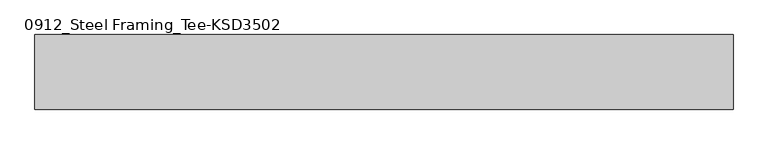
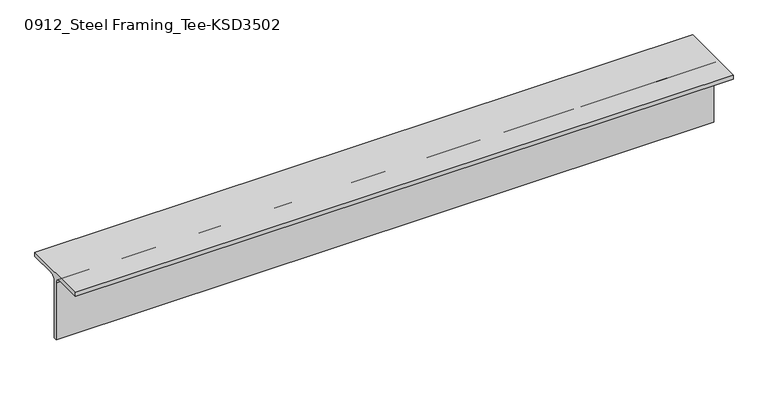
"""IFC4 building model written with IfcOpenShell, lengths in millimetres: member geometry, 0912_Steel Framing_Tee-KSD3502 : H_SB_ASB_CT-150x150x6.5x9."""

from ifc_helpers import new_model, si_unit, point, frame, frame_2d, origin, place, context, project, spatial, polyline, circle_curve, trimmed, segment, composite_curve, outline, extrude, source, transform, mapped, element, save


def member_0912_steel_framing_tee_ksd3502_cac383f4(model_context):
    return source(origin(), model_context, "Body", "SweptSolid", [
        extrude(outline(composite_curve([segment(polyline([(-75.0, 75.0), (75.0, 75.0), (75.0, 66.0), (16.25, 66.0)]), True, "CONTINUOUS"), segment(trimmed(circle_curve(frame_2d((16.25, 53.0)), 13.0), [point((16.25, 66.0))], [point((3.25, 53.0))], True, "CARTESIAN"), True, "CONTINUOUS"), segment(polyline([(3.25, 53.0), (3.25, -75.0), (-3.25, -75.0), (-3.25, 53.0)]), True, "CONTINUOUS"), segment(trimmed(circle_curve(frame_2d((-16.25, 53.0)), 13.0), [point((-3.25, 53.0))], [point((-16.25, 66.0))], True, "CARTESIAN"), True, "CONTINUOUS"), segment(polyline([(-16.25, 66.0), (-75.0, 66.0), (-75.0, 75.0)]), True, "CONTINUOUS")], self_intersect=False)), frame((-701.75, 0.0, 0.0), z_axis=(1.0, 0.0, 0.0), x_axis=(0.0, 1.0, 0.0)), (0.0, 0.0, 1.0), 1403.5),
    ])


if __name__ == "__main__":
    model = new_model("IFC4")
    model_context = context("Model", 3, world=origin())
    ifc_project = project(units=[si_unit("LENGTHUNIT", "METRE", prefix="MILLI")], contexts=[model_context])
    site = spatial("IfcSite", under=ifc_project)
    building = spatial("IfcBuilding", under=site)
    placement = place(None, origin())
    member_0912_steel_framing_tee_ksd3502_shape = member_0912_steel_framing_tee_ksd3502_cac383f4(model_context)
    element("IfcMember", 1, ObjectType="0912_Steel Framing_Tee-KSD3502 : H_SB_ASB_CT-150x150x6.5x9", at=placement, inside=building, context=model_context, shape_type="MappedRepresentation", body=[
        mapped(member_0912_steel_framing_tee_ksd3502_shape, transform((0.0, 0.0, 0.0), x_axis=(1.0, 0.0, 0.0), y_axis=(0.0, 1.0, 0.0), z_axis=(0.0, 0.0, 1.0))),
    ])
    save(model, "model.ifc")

# Revit data of these elements
# Type "0912_Steel Framing_Tee-KSD3502 : H_SB_ASB_CT-150x150x6.5x9"
#   H_WM Code_1 = "S01AA003-00001 | Main Steel Structure Fabrication Work | Shelter/Building | Light Steel - Standard (30KG/M>Weight) | Material: (   )"
#   H_WM Code_2 = "S03AA029-00001 | Main Steel Structure Erection Work | Shelter/Building | Light Steel (30KG/M>Weight) | Material: (   )"
#   H_WM Code_3 = "S01AA010-00001 | Main Steel Structure Fabrication Work | Shelter/Building | Steel Painting/Coating | for Non-Fireproofed Steel Surface, Surface Preparation, Primer, Second & Final Coat | Material: (   )"
#   H_Q'ty Cal Type Tag = "SB-Q2"
#   Width = 15.0 cm
#   Web Thickness = 0.65 cm
#   Web Fillet = 1.3 cm
#   Section Area = 23.39 cm²
#   Perimeter = 0.60 m²/m
#   Nominal Weight = 18.40 kgf/m
#   Height = 15.0 cm
#   Flange Thickness = 0.9 cm
#   Centroid Vertical = 7.5 cm
#   Centroid Horizontal = 7.5 cm
#   Length [instance default] = 1.5000 m
#   Structural Material [instance default] = Steel, 45-345
#   Warping Constant = (empty or 0)
#   Torsional Moment of Inertia = 0
#   Section Name Key = ""
#   Plastic Modulus weak axis = 0
#   Plastic Modulus strong axis = 0
#   Moment of Inertia weak axis = 0
#   Moment of Inertia strong axis = 0
#   Elastic Modulus weak axis = 0
#   Elastic Modulus strong axis = 0
#   Bolt Spacing = 0
#   Assembly Code = ""
# Element 1 (IfcMember, "0912_Steel Framing_Tee-KSD3502 : H_SB_ASB_CT-150x150x6.5x9")
#   Structural Material = none
# Materials
#   "Steel, 45-345": class "Metal", colour RGB 189 187 185, transparency 0, Description = "Steel 345 MPa", Cost = 0
